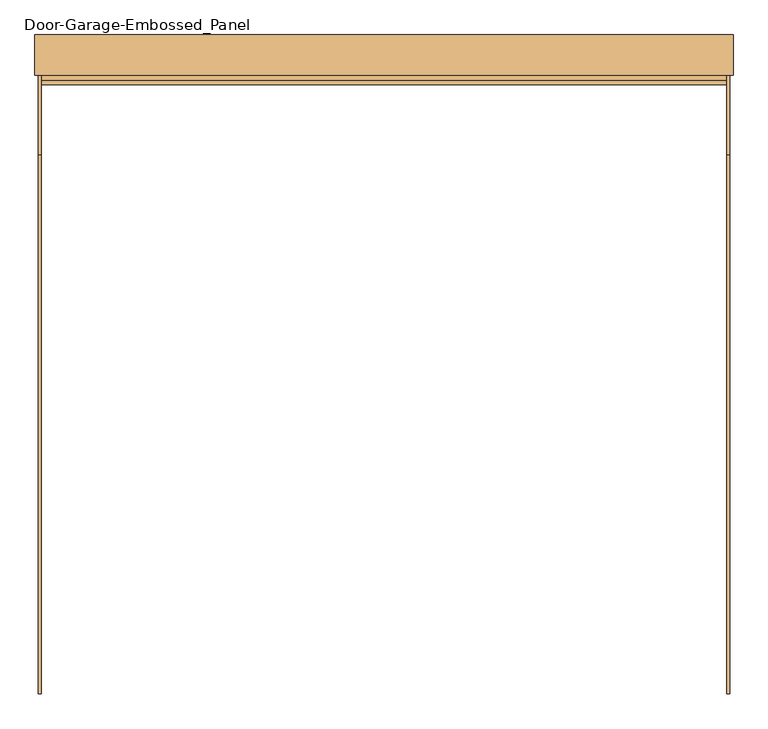
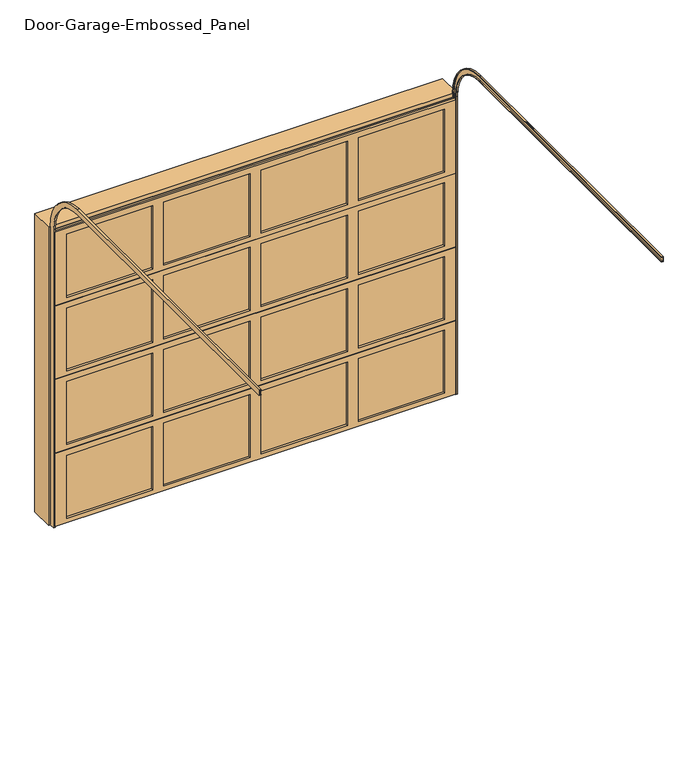
"""IFC4 building model written with IfcOpenShell, lengths in millimetres: door geometry, Door-Garage-Embossed_Panel : 108'' x 84'' 2."""

from ifc_helpers import new_model, si_unit, frame, origin, place, context, project, spatial, polyline, circle_curve, outline, extrude, faceted_brep, source, transform, mapped, element, save
from ifc_brep_helpers import plane_surface, cylinder_surface, revolved_surface, advanced_brep


def door_garage_embossed_panel_72629a66(model_context):
    return source(origin(), model_context, "Body", "SolidModel", [
        extrude(outline(polyline([(628.65, -100.0125), (628.65, -106.3625), (38.1, -106.3625), (38.1, -100.0125), (628.65, -100.0125)])), frame((0.0, 0.0, 1638.3), z_axis=(0.0, 0.0, 1.0), x_axis=(1.0, 0.0, 0.0)), (0.0, 0.0, 1.0), 457.2),
        extrude(outline(polyline([(-38.1, -100.0125), (-38.1, -106.3625), (-628.65, -106.3625), (-628.65, -100.0125), (-38.1, -100.0125)])), frame((0.0, 0.0, 1638.3), z_axis=(0.0, 0.0, 1.0), x_axis=(1.0, 0.0, 0.0)), (0.0, 0.0, 1.0), 457.2),
        extrude(outline(polyline([(1295.4, -100.0125), (1295.4, -106.3625), (704.85, -106.3625), (704.85, -100.0125), (1295.4, -100.0125)])), frame((0.0, 0.0, 1638.3), z_axis=(0.0, 0.0, 1.0), x_axis=(1.0, 0.0, 0.0)), (0.0, 0.0, 1.0), 457.2),
        extrude(outline(polyline([(-704.85, -100.0125), (-704.85, -106.3625), (-1295.4, -106.3625), (-1295.4, -100.0125), (-704.85, -100.0125)])), frame((0.0, 0.0, 1638.3), z_axis=(0.0, 0.0, 1.0), x_axis=(1.0, 0.0, 0.0)), (0.0, 0.0, 1.0), 457.2),
        faceted_brep([(1371.6, -106.3625, 2136.775), (1371.6, -122.2375, 2136.775), (1371.6, -122.2375, 1606.55), (1371.6, -100.0125, 1606.55), (1371.6, -100.0125, 1600.2), (1371.6, -84.1375, 1600.2), (1371.6, -84.1375, 2130.425), (1371.6, -106.3625, 2130.425), (-1371.6, -122.2375, 2136.775), (-1371.6, -106.3625, 2136.775), (-1371.6, -106.3625, 2130.425), (-1371.6, -84.1375, 2130.425), (-1371.6, -84.1375, 1600.2), (-1371.6, -100.0125, 1600.2), (-1371.6, -100.0125, 1606.55), (-1371.6, -122.2375, 1606.55), (704.85, -122.2375, 2095.5), (1295.4, -122.2375, 2095.5), (1295.4, -122.2375, 1638.3), (704.85, -122.2375, 1638.3), (-628.65, -122.2375, 2095.5), (-38.1, -122.2375, 2095.5), (-38.1, -122.2375, 1638.3), (-628.65, -122.2375, 1638.3), (38.1, -122.2375, 2095.5), (628.65, -122.2375, 2095.5), (628.65, -122.2375, 1638.3), (38.1, -122.2375, 1638.3), (-1295.4, -122.2375, 2095.5), (-704.85, -122.2375, 2095.5), (-704.85, -122.2375, 1638.3), (-1295.4, -122.2375, 1638.3), (1295.4, -84.1375, 2095.5), (704.85, -84.1375, 2095.5), (704.85, -84.1375, 1638.3), (1295.4, -84.1375, 1638.3), (-38.1, -84.1375, 2095.5), (-628.65, -84.1375, 2095.5), (-628.65, -84.1375, 1638.3), (-38.1, -84.1375, 1638.3), (628.65, -84.1375, 2095.5), (38.1, -84.1375, 2095.5), (38.1, -84.1375, 1638.3), (628.65, -84.1375, 1638.3), (-704.85, -84.1375, 2095.5), (-1295.4, -84.1375, 2095.5), (-1295.4, -84.1375, 1638.3), (-704.85, -84.1375, 1638.3)], [[[0, 1, 2, 3, 4, 5, 6, 7]], [[8, 9, 10, 11, 12, 13, 14, 15]], [[1, 0, 9, 8]], [[2, 1, 8, 15], [16, 17, 18, 19], [20, 21, 22, 23], [24, 25, 26, 27], [28, 29, 30, 31]], [[3, 2, 15, 14]], [[4, 3, 14, 13]], [[5, 4, 13, 12]], [[6, 5, 12, 11], [32, 33, 34, 35], [36, 37, 38, 39], [40, 41, 42, 43], [44, 45, 46, 47]], [[7, 6, 11, 10]], [[0, 7, 10, 9]], [[16, 33, 32, 17]], [[33, 16, 19, 34]], [[34, 19, 18, 35]], [[17, 32, 35, 18]], [[20, 37, 36, 21]], [[37, 20, 23, 38]], [[38, 23, 22, 39]], [[21, 36, 39, 22]], [[24, 41, 40, 25]], [[41, 24, 27, 42]], [[42, 27, 26, 43]], [[25, 40, 43, 26]], [[28, 45, 44, 29]], [[45, 28, 31, 46]], [[46, 31, 30, 47]], [[29, 44, 47, 30]]]),
        extrude(outline(polyline([(628.65, -100.0125), (628.65, -106.3625), (38.1, -106.3625), (38.1, -100.0125), (628.65, -100.0125)])), frame((0.0, 0.0, 1104.9), z_axis=(0.0, 0.0, 1.0), x_axis=(1.0, 0.0, 0.0)), (0.0, 0.0, 1.0), 457.2),
        extrude(outline(polyline([(-38.1, -100.0125), (-38.1, -106.3625), (-628.65, -106.3625), (-628.65, -100.0125), (-38.1, -100.0125)])), frame((0.0, 0.0, 1104.9), z_axis=(0.0, 0.0, 1.0), x_axis=(1.0, 0.0, 0.0)), (0.0, 0.0, 1.0), 457.2),
        extrude(outline(polyline([(1295.4, -100.0125), (1295.4, -106.3625), (704.85, -106.3625), (704.85, -100.0125), (1295.4, -100.0125)])), frame((0.0, 0.0, 1104.9), z_axis=(0.0, 0.0, 1.0), x_axis=(1.0, 0.0, 0.0)), (0.0, 0.0, 1.0), 457.2),
        extrude(outline(polyline([(-704.85, -100.0125), (-704.85, -106.3625), (-1295.4, -106.3625), (-1295.4, -100.0125), (-704.85, -100.0125)])), frame((0.0, 0.0, 1104.9), z_axis=(0.0, 0.0, 1.0), x_axis=(1.0, 0.0, 0.0)), (0.0, 0.0, 1.0), 457.2),
        faceted_brep([(1371.6, -106.3625, 1603.375), (1371.6, -122.2375, 1603.375), (1371.6, -122.2375, 1073.15), (1371.6, -100.0125, 1073.15), (1371.6, -100.0125, 1066.8), (1371.6, -84.1375, 1066.8), (1371.6, -84.1375, 1597.025), (1371.6, -106.3625, 1597.025), (-1371.6, -122.2375, 1603.375), (-1371.6, -106.3625, 1603.375), (-1371.6, -106.3625, 1597.025), (-1371.6, -84.1375, 1597.025), (-1371.6, -84.1375, 1066.8), (-1371.6, -100.0125, 1066.8), (-1371.6, -100.0125, 1073.15), (-1371.6, -122.2375, 1073.15), (704.85, -122.2375, 1562.1), (1295.4, -122.2375, 1562.1), (1295.4, -122.2375, 1104.9), (704.85, -122.2375, 1104.9), (-628.65, -122.2375, 1562.1), (-38.1, -122.2375, 1562.1), (-38.1, -122.2375, 1104.9), (-628.65, -122.2375, 1104.9), (38.1, -122.2375, 1562.1), (628.65, -122.2375, 1562.1), (628.65, -122.2375, 1104.9), (38.1, -122.2375, 1104.9), (-1295.4, -122.2375, 1562.1), (-704.85, -122.2375, 1562.1), (-704.85, -122.2375, 1104.9), (-1295.4, -122.2375, 1104.9), (1295.4, -84.1375, 1562.1), (704.85, -84.1375, 1562.1), (704.85, -84.1375, 1104.9), (1295.4, -84.1375, 1104.9), (-38.1, -84.1375, 1562.1), (-628.65, -84.1375, 1562.1), (-628.65, -84.1375, 1104.9), (-38.1, -84.1375, 1104.9), (628.65, -84.1375, 1562.1), (38.1, -84.1375, 1562.1), (38.1, -84.1375, 1104.9), (628.65, -84.1375, 1104.9), (-704.85, -84.1375, 1562.1), (-1295.4, -84.1375, 1562.1), (-1295.4, -84.1375, 1104.9), (-704.85, -84.1375, 1104.9)], [[[0, 1, 2, 3, 4, 5, 6, 7]], [[8, 9, 10, 11, 12, 13, 14, 15]], [[1, 0, 9, 8]], [[2, 1, 8, 15], [16, 17, 18, 19], [20, 21, 22, 23], [24, 25, 26, 27], [28, 29, 30, 31]], [[3, 2, 15, 14]], [[4, 3, 14, 13]], [[5, 4, 13, 12]], [[6, 5, 12, 11], [32, 33, 34, 35], [36, 37, 38, 39], [40, 41, 42, 43], [44, 45, 46, 47]], [[7, 6, 11, 10]], [[0, 7, 10, 9]], [[16, 33, 32, 17]], [[33, 16, 19, 34]], [[34, 19, 18, 35]], [[17, 32, 35, 18]], [[20, 37, 36, 21]], [[37, 20, 23, 38]], [[38, 23, 22, 39]], [[21, 36, 39, 22]], [[24, 41, 40, 25]], [[41, 24, 27, 42]], [[42, 27, 26, 43]], [[25, 40, 43, 26]], [[28, 45, 44, 29]], [[45, 28, 31, 46]], [[46, 31, 30, 47]], [[29, 44, 47, 30]]]),
        extrude(outline(polyline([(628.65, -100.0125), (628.65, -106.3625), (38.1, -106.3625), (38.1, -100.0125), (628.65, -100.0125)])), frame((0.0, 0.0, 571.5), z_axis=(0.0, 0.0, 1.0), x_axis=(1.0, 0.0, 0.0)), (0.0, 0.0, 1.0), 457.2),
        extrude(outline(polyline([(-38.1, -100.0125), (-38.1, -106.3625), (-628.65, -106.3625), (-628.65, -100.0125), (-38.1, -100.0125)])), frame((0.0, 0.0, 571.5), z_axis=(0.0, 0.0, 1.0), x_axis=(1.0, 0.0, 0.0)), (0.0, 0.0, 1.0), 457.2),
        extrude(outline(polyline([(1295.4, -100.0125), (1295.4, -106.3625), (704.85, -106.3625), (704.85, -100.0125), (1295.4, -100.0125)])), frame((0.0, 0.0, 571.5), z_axis=(0.0, 0.0, 1.0), x_axis=(1.0, 0.0, 0.0)), (0.0, 0.0, 1.0), 457.2),
        extrude(outline(polyline([(-704.85, -100.0125), (-704.85, -106.3625), (-1295.4, -106.3625), (-1295.4, -100.0125), (-704.85, -100.0125)])), frame((0.0, 0.0, 571.5), z_axis=(0.0, 0.0, 1.0), x_axis=(1.0, 0.0, 0.0)), (0.0, 0.0, 1.0), 457.2),
        faceted_brep([(1371.6, -106.3625, 1069.975), (1371.6, -122.2375, 1069.975), (1371.6, -122.2375, 539.75), (1371.6, -100.0125, 539.75), (1371.6, -100.0125, 533.4), (1371.6, -84.1375, 533.4), (1371.6, -84.1375, 1063.625), (1371.6, -106.3625, 1063.625), (-1371.6, -122.2375, 1069.975), (-1371.6, -106.3625, 1069.975), (-1371.6, -106.3625, 1063.625), (-1371.6, -84.1375, 1063.625), (-1371.6, -84.1375, 533.4), (-1371.6, -100.0125, 533.4), (-1371.6, -100.0125, 539.75), (-1371.6, -122.2375, 539.75), (704.85, -122.2375, 1028.7), (1295.4, -122.2375, 1028.7), (1295.4, -122.2375, 571.5), (704.85, -122.2375, 571.5), (-628.65, -122.2375, 1028.7), (-38.1, -122.2375, 1028.7), (-38.1, -122.2375, 571.5), (-628.65, -122.2375, 571.5), (38.1, -122.2375, 1028.7), (628.65, -122.2375, 1028.7), (628.65, -122.2375, 571.5), (38.1, -122.2375, 571.5), (-1295.4, -122.2375, 1028.7), (-704.85, -122.2375, 1028.7), (-704.85, -122.2375, 571.5), (-1295.4, -122.2375, 571.5), (1295.4, -84.1375, 1028.7), (704.85, -84.1375, 1028.7), (704.85, -84.1375, 571.5), (1295.4, -84.1375, 571.5), (-38.1, -84.1375, 1028.7), (-628.65, -84.1375, 1028.7), (-628.65, -84.1375, 571.5), (-38.1, -84.1375, 571.5), (628.65, -84.1375, 1028.7), (38.1, -84.1375, 1028.7), (38.1, -84.1375, 571.5), (628.65, -84.1375, 571.5), (-704.85, -84.1375, 1028.7), (-1295.4, -84.1375, 1028.7), (-1295.4, -84.1375, 571.5), (-704.85, -84.1375, 571.5)], [[[0, 1, 2, 3, 4, 5, 6, 7]], [[8, 9, 10, 11, 12, 13, 14, 15]], [[1, 0, 9, 8]], [[2, 1, 8, 15], [16, 17, 18, 19], [20, 21, 22, 23], [24, 25, 26, 27], [28, 29, 30, 31]], [[3, 2, 15, 14]], [[4, 3, 14, 13]], [[5, 4, 13, 12]], [[6, 5, 12, 11], [32, 33, 34, 35], [36, 37, 38, 39], [40, 41, 42, 43], [44, 45, 46, 47]], [[7, 6, 11, 10]], [[0, 7, 10, 9]], [[16, 33, 32, 17]], [[33, 16, 19, 34]], [[34, 19, 18, 35]], [[17, 32, 35, 18]], [[20, 37, 36, 21]], [[37, 20, 23, 38]], [[38, 23, 22, 39]], [[21, 36, 39, 22]], [[24, 41, 40, 25]], [[41, 24, 27, 42]], [[42, 27, 26, 43]], [[25, 40, 43, 26]], [[28, 45, 44, 29]], [[45, 28, 31, 46]], [[46, 31, 30, 47]], [[29, 44, 47, 30]]]),
        extrude(outline(polyline([(628.65, -100.0125), (628.65, -106.3625), (38.1, -106.3625), (38.1, -100.0125), (628.65, -100.0125)])), frame((0.0, 0.0, 38.1), z_axis=(0.0, 0.0, 1.0), x_axis=(1.0, 0.0, 0.0)), (0.0, 0.0, 1.0), 457.2),
        extrude(outline(polyline([(-38.1, -100.0125), (-38.1, -106.3625), (-628.65, -106.3625), (-628.65, -100.0125), (-38.1, -100.0125)])), frame((0.0, 0.0, 38.1), z_axis=(0.0, 0.0, 1.0), x_axis=(1.0, 0.0, 0.0)), (0.0, 0.0, 1.0), 457.2),
        extrude(outline(polyline([(1295.4, -100.0125), (1295.4, -106.3625), (704.85, -106.3625), (704.85, -100.0125), (1295.4, -100.0125)])), frame((0.0, 0.0, 38.1), z_axis=(0.0, 0.0, 1.0), x_axis=(1.0, 0.0, 0.0)), (0.0, 0.0, 1.0), 457.2),
        extrude(outline(polyline([(-704.85, -100.0125), (-704.85, -106.3625), (-1295.4, -106.3625), (-1295.4, -100.0125), (-704.85, -100.0125)])), frame((0.0, 0.0, 38.1), z_axis=(0.0, 0.0, 1.0), x_axis=(1.0, 0.0, 0.0)), (0.0, 0.0, 1.0), 457.2),
        faceted_brep([(1371.6, -106.3625, 536.575), (1371.6, -122.2375, 536.575), (1371.6, -122.2375, 6.35), (1371.6, -100.0125, 6.35), (1371.6, -100.0125, 0.0), (1371.6, -84.1375, 0.0), (1371.6, -84.1375, 530.225), (1371.6, -106.3625, 530.225), (-1371.6, -122.2375, 536.575), (-1371.6, -106.3625, 536.575), (-1371.6, -106.3625, 530.225), (-1371.6, -84.1375, 530.225), (-1371.6, -84.1375, 0.0), (-1371.6, -100.0125, 0.0), (-1371.6, -100.0125, 6.35), (-1371.6, -122.2375, 6.35), (704.85, -122.2375, 495.3), (1295.4, -122.2375, 495.3), (1295.4, -122.2375, 38.1), (704.85, -122.2375, 38.1), (-628.65, -122.2375, 495.3), (-38.1, -122.2375, 495.3), (-38.1, -122.2375, 38.1), (-628.65, -122.2375, 38.1), (38.1, -122.2375, 495.3), (628.65, -122.2375, 495.3), (628.65, -122.2375, 38.1), (38.1, -122.2375, 38.1), (-1295.4, -122.2375, 495.3), (-704.85, -122.2375, 495.3), (-704.85, -122.2375, 38.1), (-1295.4, -122.2375, 38.1), (1295.4, -84.1375, 495.3), (704.85, -84.1375, 495.3), (704.85, -84.1375, 38.1), (1295.4, -84.1375, 38.1), (-38.1, -84.1375, 495.3), (-628.65, -84.1375, 495.3), (-628.65, -84.1375, 38.1), (-38.1, -84.1375, 38.1), (628.65, -84.1375, 495.3), (38.1, -84.1375, 495.3), (38.1, -84.1375, 38.1), (628.65, -84.1375, 38.1), (-704.85, -84.1375, 495.3), (-1295.4, -84.1375, 495.3), (-1295.4, -84.1375, 38.1), (-704.85, -84.1375, 38.1)], [[[0, 1, 2, 3, 4, 5, 6, 7]], [[8, 9, 10, 11, 12, 13, 14, 15]], [[1, 0, 9, 8]], [[2, 1, 8, 15], [16, 17, 18, 19], [20, 21, 22, 23], [24, 25, 26, 27], [28, 29, 30, 31]], [[3, 2, 15, 14]], [[4, 3, 14, 13]], [[5, 4, 13, 12]], [[6, 5, 12, 11], [32, 33, 34, 35], [36, 37, 38, 39], [40, 41, 42, 43], [44, 45, 46, 47]], [[7, 6, 11, 10]], [[0, 7, 10, 9]], [[16, 33, 32, 17]], [[33, 16, 19, 34]], [[34, 19, 18, 35]], [[17, 32, 35, 18]], [[20, 37, 36, 21]], [[37, 20, 23, 38]], [[38, 23, 22, 39]], [[21, 36, 39, 22]], [[24, 41, 40, 25]], [[41, 24, 27, 42]], [[42, 27, 26, 43]], [[25, 40, 43, 26]], [[28, 45, 44, 29]], [[45, 28, 31, 46]], [[46, 31, 30, 47]], [[29, 44, 47, 30]]]),
        advanced_brep(
        [(1384.3, -122.2375, 0.0), (1371.6, -122.2375, 0.0), (1371.6, -119.0625, 0.0), (1381.125, -119.0625, 0.0), (1381.125, -87.3125, 0.0), (1371.6, -87.3125, 0.0), (1371.6, -84.1375, 0.0), (1384.3, -84.1375, 0.0), (1384.3, -122.2375, 2159.0), (1371.6, -122.2375, 2159.0), (1371.6, -401.6375, 2438.4), (1371.6, -2560.6375, 2438.4), (1371.6, -2560.6375, 2441.575), (1371.6, -401.6375, 2441.575), (1371.6, -119.0625, 2159.0), (1381.125, -119.0625, 2159.0), (1381.125, -401.6375, 2441.575), (1381.125, -2560.6375, 2441.575), (1381.125, -2560.6375, 2473.325), (1381.125, -401.6375, 2473.325), (1381.125, -87.3125, 2159.0), (1371.6, -87.3125, 2159.0), (1371.6, -401.6375, 2473.325), (1371.6, -2560.6375, 2473.325), (1371.6, -2560.6375, 2476.5), (1371.6, -401.6375, 2476.5), (1371.6, -84.1375, 2159.0), (1384.3, -84.1375, 2159.0), (1384.3, -401.6375, 2476.5), (1384.3, -2560.6375, 2476.5), (1384.3, -2560.6375, 2438.4), (1384.3, -401.6375, 2438.4)],
        [
            (0, 1),
            (1, 2),
            (2, 3),
            (3, 4),
            (4, 5),
            (5, 6),
            (6, 7),
            (7, 0),
            (0, 8),
            (8, 9),
            (9, 1),
            (9, 10, circle_curve(frame((1371.6, -401.6375, 2159.0), z_axis=(1.0, 0.0, 0.0), x_axis=(0.0, 1.0, 0.0)), 279.4)),
            (10, 11),
            (11, 12),
            (12, 13),
            (13, 14, circle_curve(frame((1371.6, -401.6375, 2159.0), z_axis=(-1.0, 0.0, 0.0), x_axis=(0.0, 1.0, 0.0)), 282.575)),
            (14, 2),
            (14, 15),
            (15, 3),
            (15, 16, circle_curve(frame((1381.125, -401.6375, 2159.0), z_axis=(1.0, 0.0, 0.0), x_axis=(0.0, 1.0, 0.0)), 282.575)),
            (16, 17),
            (17, 18),
            (18, 19),
            (19, 20, circle_curve(frame((1381.125, -401.6375, 2159.0), z_axis=(-1.0, 0.0, 0.0), x_axis=(0.0, 1.0, 0.0)), 314.325)),
            (20, 4),
            (20, 21),
            (21, 5),
            (21, 22, circle_curve(frame((1371.6, -401.6375, 2159.0), z_axis=(1.0, 0.0, 0.0), x_axis=(0.0, 1.0, 0.0)), 314.325)),
            (22, 23),
            (23, 24),
            (24, 25),
            (25, 26, circle_curve(frame((1371.6, -401.6375, 2159.0), z_axis=(-1.0, 0.0, 0.0), x_axis=(0.0, 1.0, 0.0)), 317.5)),
            (26, 6),
            (26, 27),
            (27, 7),
            (27, 28, circle_curve(frame((1384.3, -401.6375, 2159.0), z_axis=(1.0, 0.0, 0.0), x_axis=(0.0, 1.0, 0.0)), 317.5)),
            (28, 29),
            (29, 30),
            (30, 31),
            (31, 8, circle_curve(frame((1384.3, -401.6375, 2159.0), z_axis=(-1.0, 0.0, 0.0), x_axis=(0.0, 1.0, 0.0)), 279.4)),
            (31, 10),
            (13, 16),
            (19, 22),
            (25, 28),
            (29, 24),
            (23, 18),
            (17, 12),
            (11, 30),
        ],
        [
            plane_surface(frame((0.0, -122.2375, 0.0), z_axis=(0.0, 0.0, -1.0), x_axis=(1.0, 0.0, 0.0))),
            plane_surface(frame((1384.3, -122.2375, 0.0), z_axis=(0.0, -1.0, 0.0), x_axis=(0.0, 0.0, 1.0))),
            plane_surface(frame((1371.6, -122.2375, 0.0), z_axis=(-1.0, 0.0, 0.0), x_axis=(0.0, 0.0, 1.0))),
            plane_surface(frame((1371.6, -119.0625, 0.0), z_axis=(0.0, 1.0, 0.0), x_axis=(0.0, 0.0, 1.0))),
            plane_surface(frame((1381.125, -119.0625, 0.0), z_axis=(-1.0, 0.0, 0.0), x_axis=(0.0, 0.0, 1.0))),
            plane_surface(frame((1381.125, -87.3125, 0.0), z_axis=(0.0, -1.0, 0.0), x_axis=(0.0, 0.0, 1.0))),
            plane_surface(frame((1371.6, -87.3125, 0.0), z_axis=(-1.0, 0.0, 0.0), x_axis=(0.0, 0.0, 1.0))),
            plane_surface(frame((1371.6, -84.1375, 0.0), z_axis=(0.0, 1.0, 0.0), x_axis=(0.0, 0.0, 1.0))),
            plane_surface(frame((1384.3, -84.1375, 0.0), z_axis=(1.0, 0.0, 0.0), x_axis=(0.0, 0.0, 1.0))),
            revolved_surface(polyline([(1384.3, -122.23750000000001, 2159.0), (1371.6, -122.23750000000001, 2159.0)]), (0.0, -401.6375, 2159.0), (1.0, 0.0, 0.0)),
            cylinder_surface(frame((0.0, -401.6375, 2159.0), z_axis=(1.0, 0.0, 0.0), x_axis=(0.0, 1.0, 0.0)), 282.575),
            revolved_surface(polyline([(1381.125, -87.3125, 2159.0), (1371.6, -87.3125, 2159.0)]), (0.0, -401.6375, 2159.0), (1.0, 0.0, 0.0)),
            cylinder_surface(frame((0.0, -401.6375, 2159.0), z_axis=(1.0, 0.0, 0.0), x_axis=(0.0, 1.0, 0.0)), 317.5),
            plane_surface(frame((0.0, -2560.6375, 2438.4), z_axis=(0.0, -1.0, 0.0), x_axis=(1.0, 0.0, 0.0))),
            plane_surface(frame((1384.3, -401.6375, 2438.4), z_axis=(0.0, 0.0, -1.0), x_axis=(0.0, -1.0, 0.0))),
            plane_surface(frame((1371.6, -401.6375, 2441.575), z_axis=(0.0, 0.0, 1.0), x_axis=(0.0, -1.0, 0.0))),
            plane_surface(frame((1381.125, -401.6375, 2473.325), z_axis=(0.0, 0.0, -1.0), x_axis=(0.0, -1.0, 0.0))),
            plane_surface(frame((1371.6, -401.6375, 2476.5), z_axis=(0.0, 0.0, 1.0), x_axis=(0.0, -1.0, 0.0))),
        ],
        [
            (0, [[1, 2, 3, 4, 5, 6, 7, 8]]),
            (1, [[-1, 9, 10, 11]]),
            (2, [[-2, -11, 12, 13, 14, 15, 16, 17]]),
            (3, [[-3, -17, 18, 19]]),
            (4, [[-4, -19, 20, 21, 22, 23, 24, 25]]),
            (5, [[-5, -25, 26, 27]]),
            (6, [[-6, -27, 28, 29, 30, 31, 32, 33]]),
            (7, [[-7, -33, 34, 35]]),
            (8, [[-8, -35, 36, 37, 38, 39, 40, -9]]),
            (9, [[-12, -10, -40, 41]]),
            (10, [[-20, -18, -16, 42]]),
            (11, [[-28, -26, -24, 43]]),
            (12, [[-36, -34, -32, 44]]),
            (13, [[-38, 45, -30, 46, -22, 47, -14, 48]]),
            (14, [[-41, -39, -48, -13]]),
            (15, [[-42, -15, -47, -21]]),
            (16, [[-43, -23, -46, -29]]),
            (17, [[-44, -31, -45, -37]]),
        ],
    ),
        advanced_brep(
        [(-1384.3, -122.2375, 0.0), (-1384.3, -84.1375, 0.0), (-1371.6, -84.1375, 0.0), (-1371.6, -87.3125, 0.0), (-1381.125, -87.3125, 0.0), (-1381.125, -119.0625, 0.0), (-1371.6, -119.0625, 0.0), (-1371.6, -122.2375, 0.0), (-1384.3, -122.2375, 2159.0), (-1384.3, -401.6375, 2438.4), (-1384.3, -2560.6375, 2438.4), (-1384.3, -2560.6375, 2476.5), (-1384.3, -401.6375, 2476.5), (-1384.3, -84.1375, 2159.0), (-1371.6, -84.1375, 2159.0), (-1371.6, -401.6375, 2476.5), (-1371.6, -2560.6375, 2476.5), (-1371.6, -2560.6375, 2473.325), (-1371.6, -401.6375, 2473.325), (-1371.6, -87.3125, 2159.0), (-1381.125, -87.3125, 2159.0), (-1381.125, -401.6375, 2473.325), (-1381.125, -2560.6375, 2473.325), (-1381.125, -2560.6375, 2441.575), (-1381.125, -401.6375, 2441.575), (-1381.125, -119.0625, 2159.0), (-1371.6, -119.0625, 2159.0), (-1371.6, -401.6375, 2441.575), (-1371.6, -2560.6375, 2441.575), (-1371.6, -2560.6375, 2438.4), (-1371.6, -401.6375, 2438.4), (-1371.6, -122.2375, 2159.0)],
        [
            (0, 1),
            (1, 2),
            (2, 3),
            (3, 4),
            (4, 5),
            (5, 6),
            (6, 7),
            (7, 0),
            (0, 8),
            (8, 9, circle_curve(frame((-1384.3, -401.6375, 2159.0), z_axis=(1.0, 0.0, 0.0), x_axis=(0.0, 1.0, 0.0)), 279.4)),
            (9, 10),
            (10, 11),
            (11, 12),
            (12, 13, circle_curve(frame((-1384.3, -401.6375, 2159.0), z_axis=(-1.0, 0.0, 0.0), x_axis=(0.0, 1.0, 0.0)), 317.5)),
            (13, 1),
            (13, 14),
            (14, 2),
            (14, 15, circle_curve(frame((-1371.6, -401.6375, 2159.0), z_axis=(1.0, 0.0, 0.0), x_axis=(0.0, 1.0, 0.0)), 317.5)),
            (15, 16),
            (16, 17),
            (17, 18),
            (18, 19, circle_curve(frame((-1371.6, -401.6375, 2159.0), z_axis=(-1.0, 0.0, 0.0), x_axis=(0.0, 1.0, 0.0)), 314.325)),
            (19, 3),
            (19, 20),
            (20, 4),
            (20, 21, circle_curve(frame((-1381.125, -401.6375, 2159.0), z_axis=(1.0, 0.0, 0.0), x_axis=(0.0, 1.0, 0.0)), 314.325)),
            (21, 22),
            (22, 23),
            (23, 24),
            (24, 25, circle_curve(frame((-1381.125, -401.6375, 2159.0), z_axis=(-1.0, 0.0, 0.0), x_axis=(0.0, 1.0, 0.0)), 282.575)),
            (25, 5),
            (25, 26),
            (26, 6),
            (26, 27, circle_curve(frame((-1371.6, -401.6375, 2159.0), z_axis=(1.0, 0.0, 0.0), x_axis=(0.0, 1.0, 0.0)), 282.575)),
            (27, 28),
            (28, 29),
            (29, 30),
            (30, 31, circle_curve(frame((-1371.6, -401.6375, 2159.0), z_axis=(-1.0, 0.0, 0.0), x_axis=(0.0, 1.0, 0.0)), 279.4)),
            (31, 7),
            (31, 8),
            (12, 15),
            (18, 21),
            (24, 27),
            (30, 9),
            (10, 29),
            (28, 23),
            (22, 17),
            (16, 11),
        ],
        [
            plane_surface(frame((0.0, -122.2375, 0.0), z_axis=(0.0, 0.0, -1.0), x_axis=(1.0, 0.0, 0.0))),
            plane_surface(frame((-1384.3, -122.2375, 0.0), z_axis=(-1.0, 0.0, 0.0), x_axis=(0.0, 0.0, 1.0))),
            plane_surface(frame((-1384.3, -84.1375, 0.0), z_axis=(0.0, 1.0, 0.0), x_axis=(0.0, 0.0, 1.0))),
            plane_surface(frame((-1371.6, -84.1375, 0.0), z_axis=(1.0, 0.0, 0.0), x_axis=(0.0, 0.0, 1.0))),
            plane_surface(frame((-1371.6, -87.3125, 0.0), z_axis=(0.0, -1.0, 0.0), x_axis=(0.0, 0.0, 1.0))),
            plane_surface(frame((-1381.125, -87.3125, 0.0), z_axis=(1.0, 0.0, 0.0), x_axis=(0.0, 0.0, 1.0))),
            plane_surface(frame((-1381.125, -119.0625, 0.0), z_axis=(0.0, 1.0, 0.0), x_axis=(0.0, 0.0, 1.0))),
            plane_surface(frame((-1371.6, -119.0625, 0.0), z_axis=(1.0, 0.0, 0.0), x_axis=(0.0, 0.0, 1.0))),
            plane_surface(frame((-1371.6, -122.2375, 0.0), z_axis=(0.0, -1.0, 0.0), x_axis=(0.0, 0.0, 1.0))),
            cylinder_surface(frame((0.0, -401.6375, 2159.0), z_axis=(1.0, 0.0, 0.0), x_axis=(0.0, 1.0, 0.0)), 317.5),
            revolved_surface(polyline([(-1371.6, -87.3125, 2159.0), (-1381.125, -87.3125, 2159.0)]), (0.0, -401.6375, 2159.0), (1.0, 0.0, 0.0)),
            cylinder_surface(frame((0.0, -401.6375, 2159.0), z_axis=(1.0, 0.0, 0.0), x_axis=(0.0, 1.0, 0.0)), 282.575),
            revolved_surface(polyline([(-1371.6, -122.23750000000001, 2159.0), (-1384.3, -122.23750000000001, 2159.0)]), (0.0, -401.6375, 2159.0), (1.0, 0.0, 0.0)),
            plane_surface(frame((0.0, -2560.6375, 2438.4), z_axis=(0.0, -1.0, 0.0), x_axis=(1.0, 0.0, 0.0))),
            plane_surface(frame((-1384.3, -401.6375, 2476.5), z_axis=(0.0, 0.0, 1.0), x_axis=(0.0, -1.0, 0.0))),
            plane_surface(frame((-1371.6, -401.6375, 2473.325), z_axis=(0.0, 0.0, -1.0), x_axis=(0.0, -1.0, 0.0))),
            plane_surface(frame((-1381.125, -401.6375, 2441.575), z_axis=(0.0, 0.0, 1.0), x_axis=(0.0, -1.0, 0.0))),
            plane_surface(frame((-1371.6, -401.6375, 2438.4), z_axis=(0.0, 0.0, -1.0), x_axis=(0.0, -1.0, 0.0))),
        ],
        [
            (0, [[1, 2, 3, 4, 5, 6, 7, 8]]),
            (1, [[-1, 9, 10, 11, 12, 13, 14, 15]]),
            (2, [[-2, -15, 16, 17]]),
            (3, [[-3, -17, 18, 19, 20, 21, 22, 23]]),
            (4, [[-4, -23, 24, 25]]),
            (5, [[-5, -25, 26, 27, 28, 29, 30, 31]]),
            (6, [[-6, -31, 32, 33]]),
            (7, [[-7, -33, 34, 35, 36, 37, 38, 39]]),
            (8, [[-8, -39, 40, -9]]),
            (9, [[-18, -16, -14, 41]]),
            (10, [[-26, -24, -22, 42]]),
            (11, [[-34, -32, -30, 43]]),
            (12, [[-10, -40, -38, 44]]),
            (13, [[45, -36, 46, -28, 47, -20, 48, -12]]),
            (14, [[-41, -13, -48, -19]]),
            (15, [[-42, -21, -47, -27]]),
            (16, [[-43, -29, -46, -35]]),
            (17, [[-44, -37, -45, -11]]),
        ],
    ),
        extrude(outline(polyline([(0.0, 1371.6), (0.0, 1397.0), (2159.0, 1397.0), (2159.0, -1397.0), (0.0, -1397.0), (0.0, -1371.6), (2133.6, -1371.6), (2133.6, 1371.6), (0.0, 1371.6)])), frame((0.0, -84.1375, 0.0), z_axis=(0.0, 1.0, 0.0), x_axis=(0.0, 0.0, 1.0)), (0.0, 0.0, 1.0), 161.925),
    ])


if __name__ == "__main__":
    model = new_model("IFC4")
    model_context = context("Model", 3, world=origin())
    ifc_project = project(units=[si_unit("LENGTHUNIT", "METRE", prefix="MILLI")], contexts=[model_context])
    site = spatial("IfcSite", under=ifc_project)
    building = spatial("IfcBuilding", under=site)
    placement = place(None, origin())
    door_garage_embossed_panel_shape = door_garage_embossed_panel_72629a66(model_context)
    element("IfcDoor", 1, ObjectType="Door-Garage-Embossed_Panel : 108'' x 84'' 2", at=placement, inside=building, context=model_context, shape_type="MappedRepresentation", body=[
        mapped(door_garage_embossed_panel_shape, transform((0.0, 0.0, 0.0), x_axis=(1.0, 0.0, 0.0), y_axis=(0.0, 1.0, 0.0), z_axis=(0.0, 0.0, 1.0))),
    ])
    save(model, "model.ifc")

# Revit data of these elements
# Type "Door-Garage-Embossed_Panel : 108'' x 84'' 2"
#   Type Mark = "83"
#   COBie.Type.CreatedBy = "info@geappliances.com"
#   COBie.Type.CreatedOn = "2017-07-20T03:49:29"
#   COBie.Type.Name = "Door-Garage-Embossed_Panel_108'' x 84'' 2_83"
#   COBie.Type.Category = "23-30 10 00 : Doors"
#   COBie.Type.Description = "Door-Garage-Embossed_Panel_108'' x 84'' 2"
#   COBie.Type.Manufacturer = ""
#   COBie.Type.ModelNumber = ""
#   Analytic Construction = "Wooden"
#   COBie.Type.ReplacementCost = 0
#   Thickness = 0' - 1 1/2"
#   Thermal Resistance (R) = 0.455703 (m²·K)/W
#   Rough Width = 9' - 2"
#   Rough Height = 7' - 1"
#   Panel Height = 1' - 9"
#   Height = 7' - 0"
#   Width = 9' - 0"
#   Heat Transfer Coefficient (U) = 2.19465 W/(m²·K)
#   COBie.Type = yes
#   Panels = 4
#   Function = 1
#   Exterior Trim [instance default] = yes
#   Trim Material = Trim - White
#   Panel Material = Trim - White
#   Frame Material = Trim - White
#   Visual Light Transmittance = 0
#   Solar Heat Gain Coefficient = 0
#   Wall Closure = (empty or 0)
#   Assembly Code = ""
# Element 1 (IfcDoor, "Door-Garage-Embossed_Panel : 108'' x 84'' 2")
#   Materials on its faces: "Trim - White"
# Materials
#   "Trim - White": class "Wood", colour RGB 255 255 255, transparency 0, Cost = 0
